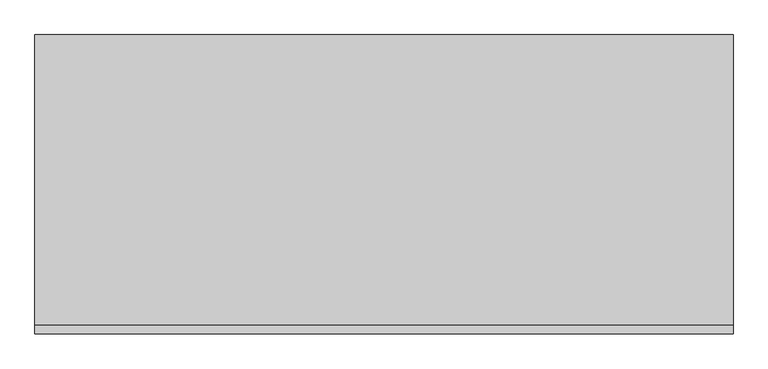
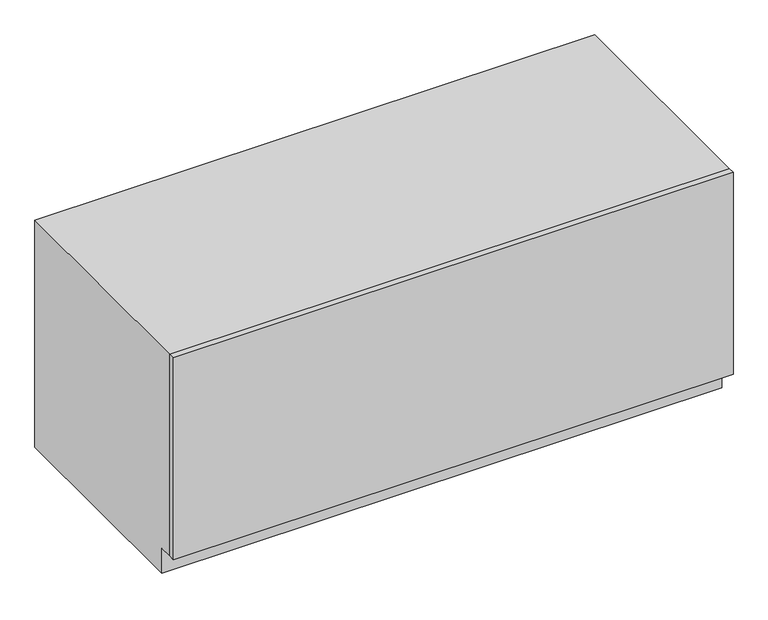
"""IFC4 building model written with IfcOpenShell, lengths in millimetres: furniture geometry, OD_CW_Base Cabinet : OD_CW_Base Cabinet."""

from ifc_helpers import new_model, si_unit, frame, origin, place, context, project, spatial, polyline, outline, extrude, source, transform, mapped, element, save


def furniture_85662207(model_context):
    return source(origin(), model_context, "Body", "SweptSolid", [
        extrude(outline(polyline([(18.7377049, -279.4), (2152.3377049, -279.4), (2152.3377049, -304.8), (18.7377049, -304.8), (18.7377049, -279.4)])), frame((0.0, 0.0, 101.6), z_axis=(0.0, 0.0, 1.0), x_axis=(1.0, 0.0, 0.0)), (0.0, 0.0, 1.0), 812.8),
        extrude(outline(polyline([(-279.4, 914.4), (609.6, 914.4), (609.6, 0.0), (-228.6, 0.0), (-228.6, 101.6), (-279.4, 101.6), (-279.4, 914.4)])), frame((18.7377049, 0.0, 0.0), z_axis=(1.0, 0.0, 0.0), x_axis=(0.0, 1.0, 0.0)), (0.0, 0.0, 1.0), 2133.6),
    ])


if __name__ == "__main__":
    model = new_model("IFC4")
    model_context = context("Model", 3, world=origin())
    ifc_project = project(units=[si_unit("LENGTHUNIT", "METRE", prefix="MILLI")], contexts=[model_context])
    site = spatial("IfcSite", under=ifc_project)
    building = spatial("IfcBuilding", under=site)
    placement = place(None, origin())
    furniture_shape = furniture_85662207(model_context)
    element("IfcFurniture", 1, ObjectType="OD_CW_Base Cabinet : OD_CW_Base Cabinet", at=placement, inside=building, context=model_context, shape_type="MappedRepresentation", body=[
        mapped(furniture_shape, transform((0.0, 0.0, 0.0), x_axis=(1.0, 0.0, 0.0), y_axis=(0.0, 1.0, 0.0), z_axis=(0.0, 0.0, 1.0))),
    ])
    save(model, "model.ifc")

# Revit data of these elements
# Type "OD_CW_Base Cabinet : OD_CW_Base Cabinet"
#   OD_CW_Width [instance default] = 2' - 10"
#   OD_CW_Length [instance default] = 8' - 0"
#   OD_CW_Height [instance default] = 2' - 3"
#   Depth = 2' - 0"
#   Height = 3' - 0"
#   Width = 4' - 0"
#   OD_CW_Material_Front Panel [instance default] = none
#   OD_CW_Material_Body [instance default] = none
# Element 1 (IfcFurniture, "OD_CW_Base Cabinet : OD_CW_Base Cabinet")
#   OD_CW_Width = 3' - 0"
#   OD_CW_Length = 7' - 0"
#   OD_CW_Height = 3' - 0"
#   OD_CW_Material_Body = PIZZA PREP
#   Materials on its faces: "PIZZA PREP", "CASEWORK"
# Materials
#   "PIZZA PREP": class "Generic", colour RGB 187 187 187, transparency 0, Cost = 0
#   "CASEWORK": class "Generic", colour RGB 181 181 181, transparency 0, Cost = 0
